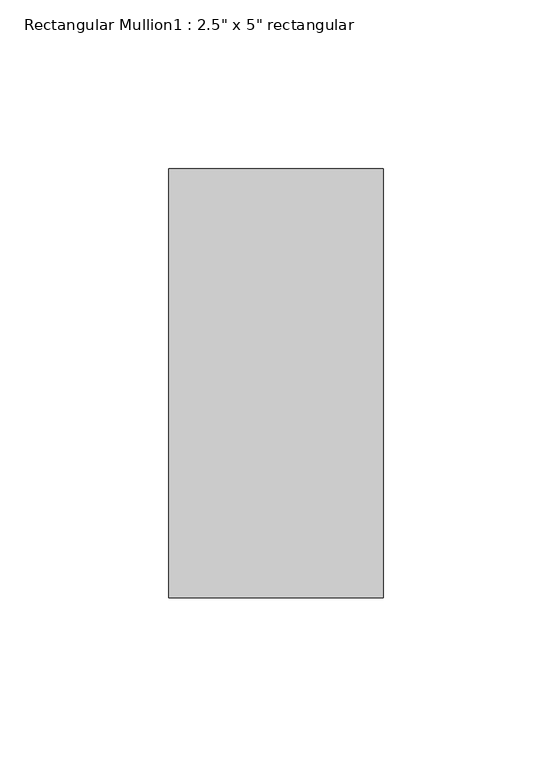
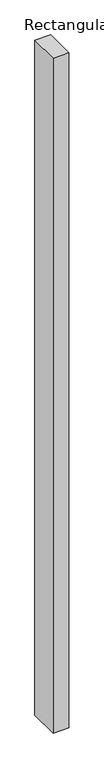
"""IFC4 building model written with IfcOpenShell, lengths in millimetres: member geometry."""

from ifc_helpers import new_model, si_unit, frame, origin, place, context, project, spatial, polyline, outline, extrude, source, transform, mapped, element, save


def member_ef0f639d(model_context):
    return source(origin(), model_context, "Body", "SweptSolid", [
        extrude(outline(polyline([(0.0, 63.5), (0.0, -63.5), (-63.5, -63.5), (-63.5, 63.5), (0.0, 63.5)])), frame((0.0, 0.0, -2884.17), z_axis=(0.0, 0.0, 1.0), x_axis=(1.0, 0.0, 0.0)), (0.0, 0.0, 1.0), 2884.17),
    ])


if __name__ == "__main__":
    model = new_model("IFC4")
    model_context = context("Model", 3, world=origin())
    ifc_project = project(units=[si_unit("LENGTHUNIT", "METRE", prefix="MILLI")], contexts=[model_context])
    site = spatial("IfcSite", under=ifc_project)
    building = spatial("IfcBuilding", under=site)
    placement = place(None, origin())
    member_shape = member_ef0f639d(model_context)
    element("IfcMember", 1, ObjectType="Rectangular Mullion1 : 2.5\" x 5\" rectangular", at=placement, inside=building, context=model_context, shape_type="MappedRepresentation", body=[
        mapped(member_shape, transform((0.0, 0.0, 0.0), x_axis=(1.0, 0.0, 0.0), y_axis=(0.0, 1.0, 0.0), z_axis=(0.0, 0.0, 1.0))),
    ])
    save(model, "model.ifc")

# Revit data of these elements
# Type "Rectangular Mullion1 : 2.5\" x 5\" rectangular"
#   built-in parameter 1007304 = 0.416667 (stored number, unit not read)
#   built-in parameter 1007301 = 0.104167 (stored number, unit not read)
#   built-in parameter 1007300 = 0.104167 (stored number, unit not read)
# Element 1 (IfcMember, "Rectangular Mullion1 : 2.5\" x 5\" rectangular")
#   Materials on its faces: "support-frame"
# Materials
#   "support-frame": class "Unassigned", colour RGB 233 233 233, transparency 0, Cost = 0
